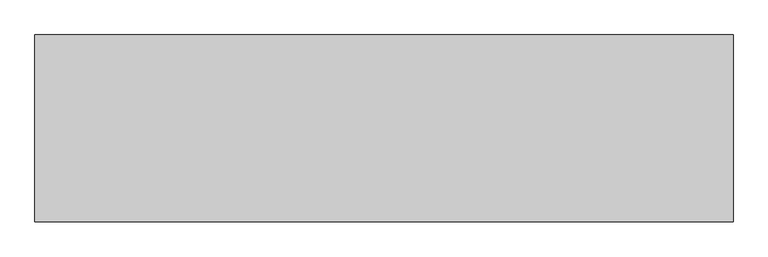
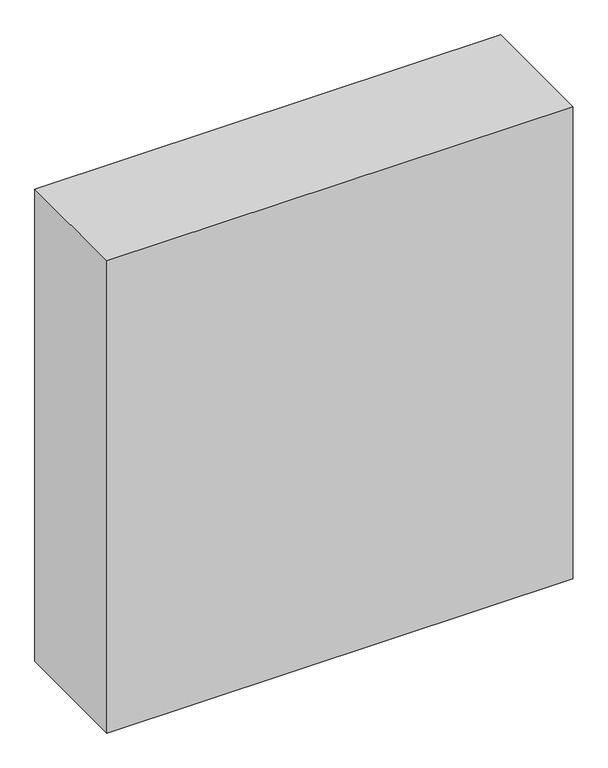
"""IFC4 building model written with IfcOpenShell, lengths in millimetres: proxy geometry, Space Planning Box_hec : Space Planning Box_hec."""

import ifcopenshell
import ifcopenshell.guid

model = None  # the IFC model being written
_history = None  # IfcOwnerHistory: only IFC2X3 demands one
_inside = {}  # id of a spatial element -> (the spatial element, [elements in it])
_under = {}  # id of a project, library or spatial element -> (it, [spatial elements below it])
_declared = {}  # id of a project -> (the project, [libraries it declares])
_typed = {}  # id of a type object -> (the type object, [elements of that type])
_made_of = {}  # id of a material, layer set ... -> (it, [elements and type objects made of it])


def new_model(schema):
    """Start an empty IFC model of exactly this schema.

    Asked for "IFC4X3", IfcOpenShell would pick the latest addendum, in which some entities
    have other attributes; the version numbers below select the first issue.
    IFC2X3 requires an IfcOwnerHistory on every rooted entity: one is made here for all.
    """
    global model, _history
    if schema == "IFC4X3":
        model = ifcopenshell.file(schema_version=(4, 3, 0, 0))
    else:
        model = ifcopenshell.file(schema=schema)
    _inside.clear()
    _under.clear()
    _declared.clear()
    _typed.clear()
    _made_of.clear()
    _history = None
    if model.schema == "IFC2X3":
        org = make("IfcOrganization", Name="unknown")
        user = make(
            "IfcPersonAndOrganization",
            ThePerson=make("IfcPerson", FamilyName="unknown"),
            TheOrganization=org,
        )
        app = make(
            "IfcApplication",
            ApplicationDeveloper=org,
            Version="unknown",
            ApplicationFullName="unknown",
            ApplicationIdentifier="unknown",
        )
        _history = make(
            "IfcOwnerHistory",
            OwningUser=user,
            OwningApplication=app,
            ChangeAction="ADDED",
            CreationDate=0,
        )
    return model


def make(cls, **values):
    """One entity of the class cls with the attributes given. An attribute that is None is left unset."""
    return model.create_entity(
        cls, **{name: value for name, value in values.items() if value is not None}
    )


def rooted(cls, **values):
    """An entity with a GlobalId (a new one), such as an element, a storey or a relation."""
    return make(cls, GlobalId=ifcopenshell.guid.new(), OwnerHistory=_history, **values)


def si_unit(unit_type, name, prefix=None):
    """IfcSIUnit, for example si_unit("LENGTHUNIT", "METRE", prefix="MILLI")."""
    return make("IfcSIUnit", UnitType=unit_type, Prefix=prefix, Name=name)


def assignment(units):
    """IfcUnitAssignment: the units of a project."""
    return None if units is None else make("IfcUnitAssignment", Units=units)


def point(xyz):
    """IfcCartesianPoint."""
    return None if xyz is None else make("IfcCartesianPoint", Coordinates=xyz)


def direction(xyz):
    """IfcDirection."""
    return None if xyz is None else make("IfcDirection", DirectionRatios=xyz)


def frame(location, z_axis=None, x_axis=None):
    """IfcAxis2Placement3D, a coordinate frame: its origin and axes. An axis left out is left unset."""
    return make(
        "IfcAxis2Placement3D",
        Location=point(location),
        Axis=direction(z_axis),
        RefDirection=direction(x_axis),
    )


def origin():
    """The frame at (0, 0, 0) with its axes left unset."""
    return frame((0.0, 0.0, 0.0))


def origin_with_axes():
    """The frame at (0, 0, 0) with the z axis (0, 0, 1) and the x axis (1, 0, 0) written out."""
    return frame((0.0, 0.0, 0.0), z_axis=(0.0, 0.0, 1.0), x_axis=(1.0, 0.0, 0.0))


def place(relative_to, where):
    """IfcLocalPlacement: puts the frame where relative to a parent placement (None: the world)."""
    return make(
        "IfcLocalPlacement", PlacementRelTo=relative_to, RelativePlacement=where
    )


def context(
    kind, dimensions, precision=None, world=None, true_north=None, identifier=None
):
    """IfcGeometricRepresentationContext, for example the 3D "Model" context."""
    return make(
        "IfcGeometricRepresentationContext",
        ContextIdentifier=identifier,
        ContextType=kind,
        CoordinateSpaceDimension=dimensions,
        Precision=precision,
        WorldCoordinateSystem=world,
        TrueNorth=true_north,
    )


def project(units=None, contexts=None):
    """IfcProject with its units and contexts."""
    return rooted(
        "IfcProject",
        Name="project",
        RepresentationContexts=contexts,
        UnitsInContext=assignment(units),
    )


def spatial(cls, under=None, at=None, **own):
    """A site, building, storey or space (cls), placed at a placement, below another one or the project."""
    s = rooted(cls, ObjectPlacement=at, **own)
    if under is not None:
        _under.setdefault(under.id(), (under, []))[1].append(s)
    return s


def polyline(points):
    """IfcPolyline through the points."""
    return make("IfcPolyline", Points=[point(p) for p in points])


def outline(outer, holes=None, kind="AREA"):
    """IfcArbitraryClosedProfileDef: a profile drawn as a closed curve; with holes, ...WithVoids."""
    if holes is None:
        return make("IfcArbitraryClosedProfileDef", ProfileType=kind, OuterCurve=outer)
    return make(
        "IfcArbitraryProfileDefWithVoids",
        ProfileType=kind,
        OuterCurve=outer,
        InnerCurves=holes,
    )


def extrude(swept, where, along, depth):
    """IfcExtrudedAreaSolid: the profile swept, set in the frame where, extruded along a direction by depth."""
    return make(
        "IfcExtrudedAreaSolid",
        SweptArea=swept,
        Position=where,
        ExtrudedDirection=direction(along),
        Depth=depth,
    )


def shape(context_of_items, identifier, shape_type, items):
    """IfcShapeRepresentation: the items that make up one representation, for example the "Body"."""
    return make(
        "IfcShapeRepresentation",
        ContextOfItems=context_of_items,
        RepresentationIdentifier=identifier,
        RepresentationType=shape_type,
        Items=items,
    )


def source(mapping_origin, context_of_items, identifier, shape_type, items):
    """IfcRepresentationMap: a shape defined once, which mapped items show again and again."""
    return make(
        "IfcRepresentationMap",
        MappingOrigin=mapping_origin,
        MappedRepresentation=shape(context_of_items, identifier, shape_type, items),
    )


def transform(
    local_origin,
    x_axis=None,
    y_axis=None,
    z_axis=None,
    scale=None,
    scale2=None,
    scale3=None,
    uniform=True,
):
    """IfcCartesianTransformationOperator3D, or its non-uniform kind. x_axis, y_axis, z_axis: its Axis1, 2, 3."""
    if uniform:
        return make(
            "IfcCartesianTransformationOperator3D",
            Axis1=direction(x_axis),
            Axis2=direction(y_axis),
            LocalOrigin=point(local_origin),
            Scale=scale,
            Axis3=direction(z_axis),
        )
    return make(
        "IfcCartesianTransformationOperator3DnonUniform",
        Axis1=direction(x_axis),
        Axis2=direction(y_axis),
        LocalOrigin=point(local_origin),
        Scale=scale,
        Axis3=direction(z_axis),
        Scale2=scale2,
        Scale3=scale3,
    )


def mapped(mapping_source, mapping_target):
    """IfcMappedItem: shows the shape of a source again, moved by a transform."""
    return make(
        "IfcMappedItem", MappingSource=mapping_source, MappingTarget=mapping_target
    )


def made_of(thing, what):
    """Note that an element or type object is made of a material, layer set ...; save() writes the relation."""
    if what is not None:
        _made_of.setdefault(what.id(), (what, []))[1].append(thing)
    return thing


def element(
    cls,
    number,
    at=None,
    inside=None,
    cuts=None,
    type_object=None,
    material=None,
    context=None,
    identifier="Body",
    shape_type=None,
    held_by="IfcProductDefinitionShape",
    body=None,
    shapes=None,
    **own,
):
    """One element of the class cls, such as IfcWall. Its Tag is "e" and its number.

    at: its placement. inside: the storey or other place that contains it. cuts: it is an
    opening in that element (IfcRelVoidsElement). A single representation is given by context,
    identifier, shape_type and body (its items); several are given by shapes. held_by: the class
    of the entity that holds the representations. save() writes the other relations.
    """
    e = rooted(cls, Tag="e%d" % number, ObjectPlacement=at, **own)
    if body is not None:
        shapes = [shape(context, identifier, shape_type, body)]
    if shapes is not None:
        e.Representation = make(held_by, Representations=shapes)
    if inside is not None:
        _inside.setdefault(inside.id(), (inside, []))[1].append(e)
    if cuts is not None:
        rooted(
            "IfcRelVoidsElement", RelatingBuildingElement=cuts, RelatedOpeningElement=e
        )
    if type_object is not None:
        _typed.setdefault(type_object.id(), (type_object, []))[1].append(e)
    return made_of(e, material)


def aggregate(whole, parts):
    """IfcRelAggregates: a whole, such as a stair, and the parts it consists of."""
    return rooted("IfcRelAggregates", RelatingObject=whole, RelatedObjects=parts)


def save(model, path):
    """Write the relations noted so far, then the file.

    IfcRelAggregates (storeys below a building ...), IfcRelContainedInSpatialStructure (elements
    in a storey), IfcRelDefinesByType, IfcRelAssociatesMaterial and IfcRelDeclares: one each for
    every whole, place, type object, material and project.
    """
    for whole, parts in _under.values():
        aggregate(whole, parts)
    for where, things in _inside.values():
        rooted(
            "IfcRelContainedInSpatialStructure",
            RelatedElements=things,
            RelatingStructure=where,
        )
    for kind, things in _typed.values():
        rooted("IfcRelDefinesByType", RelatedObjects=things, RelatingType=kind)
    for what, things in _made_of.values():
        rooted("IfcRelAssociatesMaterial", RelatedObjects=things, RelatingMaterial=what)
    for by, libraries in _declared.values():
        rooted("IfcRelDeclares", RelatingContext=by, RelatedDefinitions=libraries)
    model.write(path)


def generic_models_85897e09(model_context):
    return source(origin(), model_context, "Body", "SweptSolid", [
        extrude(outline(polyline([(2800.0, 750.0), (2800.0, -750.0), (-2800.0, -750.0), (-2800.0, 750.0), (2800.0, 750.0)])), origin_with_axes(), (0.0, 0.0, 1.0), 6000.0),
    ])


if __name__ == "__main__":
    model = new_model("IFC4")
    model_context = context("Model", 3, world=origin())
    ifc_project = project(units=[si_unit("LENGTHUNIT", "METRE", prefix="MILLI")], contexts=[model_context])
    site = spatial("IfcSite", under=ifc_project)
    building = spatial("IfcBuilding", under=site)
    placement = place(None, origin())
    generic_models_shape = generic_models_85897e09(model_context)
    element("IfcBuildingElementProxy", 1, Name="Space Planning Box_hec : Space Planning Box_hec", ObjectType="Space Planning Box_hec : Space Planning Box_hec", at=placement, inside=building, context=model_context, shape_type="MappedRepresentation", body=[
        mapped(generic_models_shape, transform((0.0, 0.0, 0.0), x_axis=(1.0, 0.0, 0.0), y_axis=(0.0, 1.0, 0.0), z_axis=(0.0, 0.0, 1.0))),
    ])
    save(model, "model.ifc")

# Revit data of these elements
# Type "Space Planning Box_hec : Space Planning Box_hec"
#   Type Comments = "..."
#   Room Name [instance default] = "?"
#   Interior Finish [instance default] = ""
#   Exterior Finish [instance default] = ""
#   Department [instance default] = ""
#   Assembly Code = "..."
#   Width [instance default] = 1524 mm
#   Program Area [instance default] = 0 m²
#   Length [instance default] = 1524 mm
#   Height [instance default] = 1524 mm
#   Area [instance default] = 2.32258 m²
#   Fill Color [instance default] = Cyan
#   Default Elevation = 0
# Element 1 (IfcBuildingElementProxy, "Space Planning Box_hec : Space Planning Box_hec")
#   Room Name = "Shower Room (M)"
#   Interior Finish = "IF5"
#   Exterior Finish = "EF1"
#   Department = "AR"
#   Width = 5600 mm
#   Program Area = 31.5 m²
#   Length = 1500 mm
#   Height = 6000 mm
#   Area = 8.4 m²
#   Fill Color = Lavender
#   Materials on its faces: "Lavender"
# Materials
#   "Cyan": class "Generic", colour RGB 0 255 255, transparency 0.2, Cost = 0
#   "Lavender": class "Generic", colour RGB 186 85 211, transparency 0.2, Cost = 0
